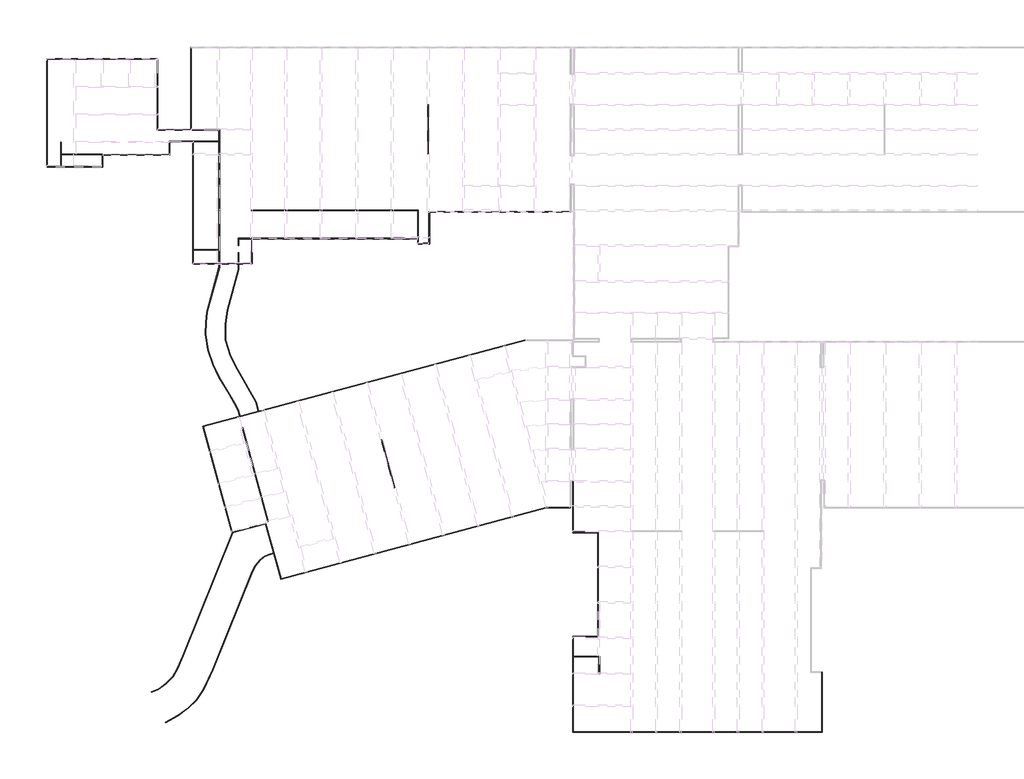
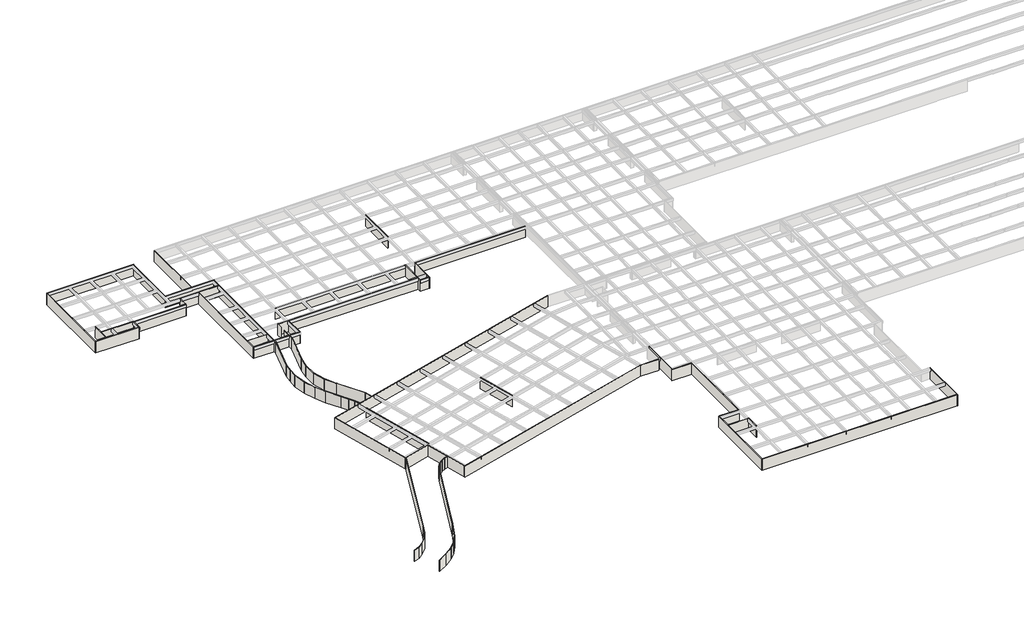
# One storey, part 1 of 14: 79 walls.
# Revit data of these elements (continued)
# Area at (93873.842, -192410.706) mm, upper offset 0 mm, lower offset 0 mm
#   Number = "228"
#   Name = "fire_compart"
# Area, not placed, upper offset 0 mm, lower offset 0 mm
#   Number = "66"
#   Name = "main_building"
# Area, not placed, upper offset 0 mm, lower offset 0 mm
#   Number = "126"
#   Name = "fire_compart"
# Area, not placed, upper offset 0 mm, lower offset 0 mm
#   Number = "83"
#   Name = "fire_compart"
# Area, not placed, upper offset 0 mm, lower offset 0 mm
#   Number = "84"
#   Name = "main_building"
# Area at (-21877.414, -126722.337) mm, upper offset 0 mm, lower offset 0 mm
#   Number = "224"
#   Name = "fire_compart"
# Area, not placed, upper offset 0 mm, lower offset 0 mm
#   Number = "150"
#   Name = "main_building"
# Area, not placed, upper offset 0 mm, lower offset 0 mm
#   Number = "127"
#   Name = "fire_compart"
# Area, not placed, upper offset 0 mm, lower offset 0 mm
#   Number = "7"
#   Name = "fire_compart_5"
# Area, not placed, upper offset 0 mm, lower offset 0 mm
#   Number = "175"
#   Name = "main_building"
# Area, not placed, upper offset 0 mm, lower offset 0 mm
#   Number = "176"
#   Name = "main_building"
# Area, not placed, upper offset 0 mm, lower offset 0 mm
#   Number = "194"
#   Name = "fire_compart"
# Area, not placed, upper offset 0 mm, lower offset 0 mm
#   Number = "128"
#   Name = "fire_compart"
# Area, not placed, upper offset 0 mm, lower offset 0 mm
#   Number = "162"
#   Name = "main_building"
# Area, not placed, upper offset 0 mm, lower offset 0 mm
#   Number = "129"
#   Name = "fire_compart"
# Area, not placed, upper offset 0 mm, lower offset 0 mm
#   Number = "151"
#   Name = "main_building"
# Area, not placed, upper offset 0 mm, lower offset 0 mm
#   Number = "187"
#   Name = "main_building"
# Area, not placed, upper offset 0 mm, lower offset 0 mm
#   Number = "130"
#   Name = "fire_compart"
# Area, not placed, upper offset 0 mm, lower offset 0 mm
#   Number = "109"
#   Name = "main_building"
# Area, not placed, upper offset 0 mm, lower offset 0 mm
#   Number = "195"
#   Name = "面积"
# Area, not placed, upper offset 0 mm, lower offset 0 mm
#   Number = "196"
#   Name = "fire_compart"
# Area, not placed, upper offset 0 mm, lower offset 0 mm
#   Number = "67"
#   Name = "fire_compart"
# Area, not placed, upper offset 0 mm, lower offset 0 mm
#   Number = "112"
#   Name = "main_building"
# Area, not placed, upper offset 0 mm, lower offset 0 mm
#   Number = "197"
#   Name = "fire_compart"
# Area, not placed, upper offset 0 mm, lower offset 0 mm
#   Number = "198"
#   Name = "fire_compart"
# Area, not placed, upper offset 0 mm, lower offset 0 mm
#   Number = "131"
#   Name = "fire_compart"
# Area, not placed, upper offset 0 mm, lower offset 0 mm
#   Number = "199"
#   Name = "fire_compart"
# Area, not placed, upper offset 0 mm, lower offset 0 mm
#   Number = "68"
#   Name = "fire_compart"
# Area, not placed, upper offset 0 mm, lower offset 0 mm
#   Number = "152"
#   Name = "main_building"
# Area, not placed, upper offset 0 mm, lower offset 0 mm
#   Number = "132"
#   Name = "fire_compart"
# Area, not placed, upper offset 0 mm, lower offset 0 mm
#   Number = "1"
#   Name = "面积"
# Area, not placed, upper offset 0 mm, lower offset 0 mm
#   Number = "2"
#   Name = "防火区域1"
# Area, not placed, upper offset 0 mm, lower offset 0 mm
#   Number = "188"
#   Name = "main_building"
# Area, not placed, upper offset 0 mm, lower offset 0 mm
#   Number = "133"
#   Name = "fire_compart"
# Area, not placed, upper offset 0 mm, lower offset 0 mm
#   Number = "144"
#   Name = "fire_compart"
# Area, not placed, upper offset 0 mm, lower offset 0 mm
#   Number = "200"
#   Name = "fire_compart"
# Area, not placed, upper offset 0 mm, lower offset 0 mm
#   Number = "201"
#   Name = "fire_compart"
# Area, not placed, upper offset 0 mm, lower offset 0 mm
#   Number = "202"
#   Name = "fire_compart"
# Area, not placed, upper offset 0 mm, lower offset 0 mm
#   Number = "134"
#   Name = "fire_compart"
# Area, not placed, upper offset 0 mm, lower offset 0 mm
#   Number = "203"
#   Name = "fire_compart"
# Area, not placed, upper offset 0 mm, lower offset 0 mm
#   Number = "25"
#   Name = "fire_compart"
# Area, not placed, upper offset 0 mm, lower offset 0 mm
#   Number = "26"
#   Name = "fire_compart"
# Area, not placed, upper offset 0 mm, lower offset 0 mm
#   Number = "27"
#   Name = "fire_compart"
# Area at (173589.182, -137755.994) mm, upper offset 0 mm, lower offset 0 mm
#   Number = "230"
#   Name = "fire_compart"
# Area at (80517.587, -167193.148) mm, upper offset 0 mm, lower offset 0 mm
#   Number = "231"
#   Name = "main_building"
# Area, not placed, upper offset 0 mm, lower offset 0 mm
#   Number = "69"
#   Name = "fire_compart"
# Area, not placed, upper offset 0 mm, lower offset 0 mm
#   Number = "105"
#   Name = "main_building"
# Area, not placed, upper offset 0 mm, lower offset 0 mm
#   Number = "113"
#   Name = "main_building"
# Area, not placed, upper offset 0 mm, lower offset 0 mm
#   Number = "153"
#   Name = "main_building"
# Area, not placed, upper offset 0 mm, lower offset 0 mm
#   Number = "177"
#   Name = "main_building"
# Area, not placed, upper offset 0 mm, lower offset 0 mm
#   Number = "135"
#   Name = "fire_compart"
# Area, not placed, upper offset 0 mm, lower offset 0 mm
#   Number = "189"
#   Name = "main_building"
# Area at (-63949.789, -174826.625) mm, upper offset 0 mm, lower offset 0 mm
#   Number = "232"
#   Name = "main_building"
# Area, not placed, upper offset 0 mm, lower offset 0 mm
#   Number = "233"
#   Name = "main_building"
# Area at (102064.836, -132989.745) mm, upper offset 0 mm, lower offset 0 mm
#   Number = "229"
#   Name = "fire_compart"
# Area, not placed, upper offset 0 mm, lower offset 0 mm
#   Number = "85"
#   Name = "fire_compart"
# Area, not placed, upper offset 0 mm, lower offset 0 mm
#   Number = "86"
#   Name = "main_building"
# Area, not placed, upper offset 0 mm, lower offset 0 mm
#   Number = "87"
#   Name = "main_building"
# Area, not placed, upper offset 0 mm, lower offset 0 mm
#   Number = "216"
#   Name = "main_building"
# Area, not placed, upper offset 0 mm, lower offset 0 mm
#   Number = "136"
#   Name = "fire_compart"
# Room, not placed, phase "新构造", upper offset 0 mm, lower offset 0 mm
#   Number = "8"
#   Name = "客餐厅"
# Area, not placed, upper offset 0 mm, lower offset 0 mm
#   Number = "217"
#   Name = "main_building"
# Area, not placed, upper offset 0 mm, lower offset 0 mm
#   Number = "70"
#   Name = "main_building"
# Area, not placed, upper offset 0 mm, lower offset 0 mm
#   Number = "156"
#   Name = "fire_compart"
# Area, not placed, upper offset 0 mm, lower offset 0 mm
#   Number = "154"
#   Name = "main_building"
# Area, not placed, upper offset 0 mm, lower offset 0 mm
#   Number = "190"
#   Name = "main_building"
# Area, not placed, upper offset 0 mm, lower offset 0 mm
#   Number = "114"
#   Name = "main_building"
# Area, not placed, upper offset 0 mm, lower offset 0 mm
#   Number = "218"
#   Name = "main_building"
# Area, not placed, upper offset 0 mm, lower offset 0 mm
#   Number = "8"
#   Name = "fire_compart_6"
# Area, not placed, upper offset 0 mm, lower offset 0 mm
#   Number = "137"
#   Name = "fire_compart"
# Area, not placed, upper offset 0 mm, lower offset 0 mm
#   Number = "178"
#   Name = "main_building"
# Area at (139335.498, -199826.366) mm, upper offset 0 mm, lower offset 0 mm
#   Number = "235"
#   Name = "main_building"
# Area at (-6636.96, -166023.589) mm, upper offset 0 mm, lower offset 0 mm
#   Number = "236"
#   Name = "main_building"
# Area, not placed, upper offset 0 mm, lower offset 0 mm
#   Number = "163"
#   Name = "main_building"
# Area, not placed, upper offset 0 mm, lower offset 0 mm
#   Number = "138"
#   Name = "fire_compart"
# Area, not placed, upper offset 0 mm, lower offset 0 mm
#   Number = "3"
#   Name = "fire_compart_1"
# Area, not placed, upper offset 0 mm, lower offset 0 mm
#   Number = "168"
#   Name = "fire_compart"
# Area, not placed, upper offset 0 mm, lower offset 0 mm
#   Number = "213"
#   Name = "fire_compart"
# Area, not placed, upper offset 0 mm, lower offset 0 mm
#   Number = "139"
#   Name = "fire_compart"
# Area, not placed, upper offset 0 mm, lower offset 0 mm
#   Number = "71"
#   Name = "fire_compart"
# Room, not placed, phase "新构造", upper offset 0 mm, lower offset 0 mm
#   Number = "11"
#   Name = "房间"
# Area, not placed, upper offset 0 mm, lower offset 0 mm
#   Number = "140"
#   Name = "fire_compart"
# Area, not placed, upper offset 0 mm, lower offset 0 mm
#   Number = "191"
#   Name = "main_building"
# Area, not placed, upper offset 0 mm, lower offset 0 mm
#   Number = "155"
#   Name = "main_building"
# Area, not placed, upper offset 0 mm, lower offset 0 mm
#   Number = "106"
#   Name = "main_building"
# Room, not placed, phase "新构造", upper offset 0 mm, lower offset 0 mm
#   Number = "12"
#   Name = "房间"
# Area, not placed, upper offset 0 mm, lower offset 0 mm
#   Number = "110"
#   Name = "main_building"
# Area, not placed, upper offset 0 mm, lower offset 0 mm
#   Number = "115"
#   Name = "main_building"
# Area, not placed, upper offset 0 mm, lower offset 0 mm
#   Number = "141"
#   Name = "fire_compart"
# Area, not placed, upper offset 0 mm, lower offset 0 mm
#   Number = "100"
#   Name = "main_building"
# Area, not placed, upper offset 0 mm, lower offset 0 mm
#   Number = "179"
#   Name = "main_building"
# Room, not placed, phase "新构造", upper offset 0 mm, lower offset 0 mm
#   Number = "13"
#   Name = "房间"
# Room, not placed, phase "新构造", upper offset 0 mm, lower offset 0 mm
#   Number = "14"
#   Name = "房间"
# Area, not placed, upper offset 0 mm, lower offset 0 mm
#   Number = "72"
#   Name = "main_building"
# Room, not placed, phase "新构造", upper offset 0 mm, lower offset 0 mm
#   Number = "15"
#   Name = "房间"
# Area, not placed, upper offset 0 mm, lower offset 0 mm
#   Number = "88"
#   Name = "fire_compart"
# Area, not placed, upper offset 0 mm, lower offset 0 mm
#   Number = "192"
#   Name = "main_building"
# Room, not placed, phase "新构造", upper offset 0 mm, lower offset 0 mm
#   Number = "16"
#   Name = "房间"
# Area, not placed, upper offset 0 mm, lower offset 0 mm
#   Number = "28"
#   Name = "面积"
# Area, not placed, upper offset 0 mm, lower offset 0 mm
#   Number = "211"
#   Name = "fire_compart"
# Area, not placed, upper offset 0 mm, lower offset 0 mm
#   Number = "73"
#   Name = "fire_compart"
# Area, not placed, upper offset 0 mm, lower offset 0 mm
#   Number = "116"
#   Name = "main_building"
# Area, not placed, upper offset 0 mm, lower offset 0 mm
#   Number = "101"
#   Name = "main_building"
# Area, not placed, upper offset 0 mm, lower offset 0 mm
#   Number = "193"
#   Name = "main_building"
# Room, not placed, phase "新构造", upper offset 0 mm, lower offset 0 mm
#   Number = "17"
#   Name = "房间"
# Area, not placed, upper offset 0 mm, lower offset 0 mm
#   Number = "30"
#   Name = "main_building"
# Area, not placed, upper offset 0 mm, lower offset 0 mm
#   Number = "143"
#   Name = "fire_compart"
# Area at (34982.03, -197012.884) mm, upper offset 0 mm, lower offset 0 mm
#   Number = "227"
#   Name = "fire_compart"
# Area, not placed, upper offset 0 mm, lower offset 0 mm
#   Number = "180"
#   Name = "main_building"
# Area, not placed, upper offset 0 mm, lower offset 0 mm
#   Number = "212"
#   Name = "fire_compart"
# Area, not placed, upper offset 0 mm, lower offset 0 mm
#   Number = "89"
#   Name = "main_building"
# Area, not placed, upper offset 0 mm, lower offset 0 mm
#   Number = "75"
#   Name = "main_building"
# Area, not placed, upper offset 0 mm, lower offset 0 mm
#   Number = "111"
#   Name = "main_building"
# Area, not placed, upper offset 0 mm, lower offset 0 mm
#   Number = "90"
#   Name = "fire_compart"
# Area, not placed, upper offset 0 mm, lower offset 0 mm
#   Number = "76"
#   Name = "main_building"
# Area, not placed, upper offset 0 mm, lower offset 0 mm
#   Number = "145"
#   Name = "fire_compart"
# Area, not placed, upper offset 0 mm, lower offset 0 mm
#   Number = "146"
#   Name = "fire_compart"
# Area, not placed, upper offset 0 mm, lower offset 0 mm
#   Number = "147"
#   Name = "fire_compart"
# Area, not placed, upper offset 0 mm, lower offset 0 mm
#   Number = "214"
#   Name = "fire_compart"
# Area, not placed, upper offset 0 mm, lower offset 0 mm
#   Number = "117"
#   Name = "main_building"
# Area, not placed, upper offset 0 mm, lower offset 0 mm
#   Number = "4"
#   Name = "fire_compart_2"
# Area at (-62904.455, -237299.426) mm, upper offset 0 mm, lower offset 0 mm
#   Number = "234"
#   Name = "main_building"
# Area, not placed, upper offset 0 mm, lower offset 0 mm
#   Number = "77"
#   Name = "main_building"
# Area, not placed, upper offset 0 mm, lower offset 0 mm
#   Number = "181"
#   Name = "main_building"
# Area, not placed, upper offset 0 mm, lower offset 0 mm
#   Number = "159"
#   Name = "fire_compart"
# Area, not placed, upper offset 0 mm, lower offset 0 mm
#   Number = "78"
#   Name = "main_building"
# Area, not placed, upper offset 0 mm, lower offset 0 mm
#   Number = "79"
#   Name = "main_building"
# Area, not placed, upper offset 0 mm, lower offset 0 mm
#   Number = "29"
#   Name = "main_building"
